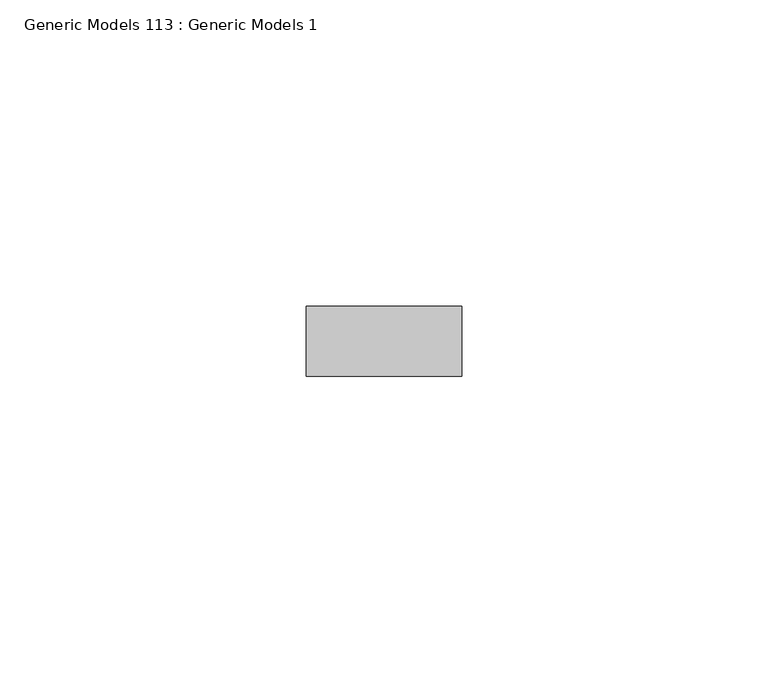
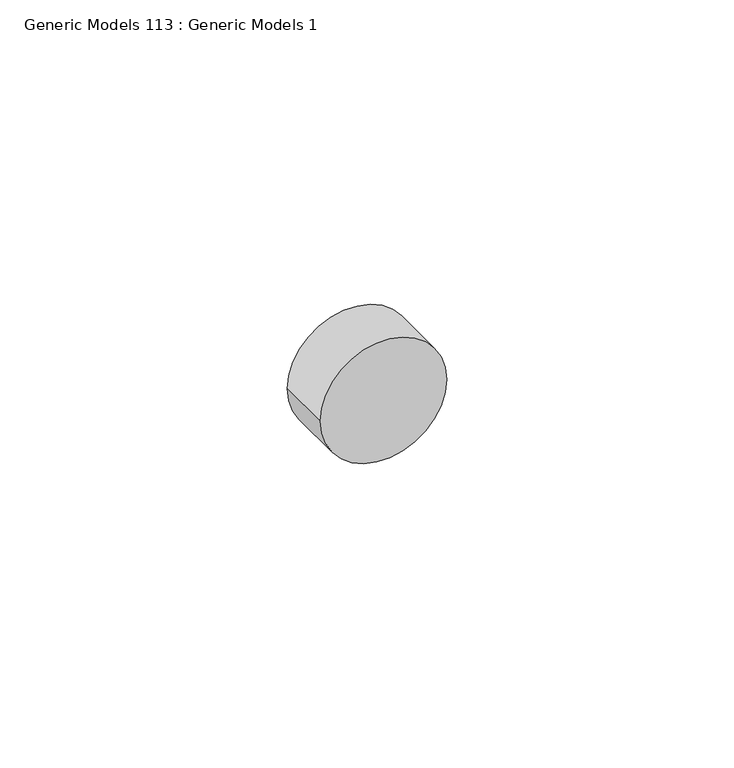
"""IFC4 building model written with IfcOpenShell, lengths in millimetres: proxy geometry, Generic Models 113 : Generic Models 1."""

from ifc_helpers import new_model, si_unit, point, frame, frame_2d, origin, place, context, project, spatial, circle_curve, trimmed, segment, composite_curve, outline, extrude, source, transform, mapped, element, save


def generic_models_113_generic_models_1_33cf204b(model_context):
    return source(origin(), model_context, "Body", "SweptSolid", [
        extrude(outline(composite_curve([segment(trimmed(circle_curve(frame_2d((37860.4162436, 6848.7828124)), 12.7), [point((37860.4162436, 6836.0828124))], [point((37860.4162436, 6861.4828124))], False, "CARTESIAN"), True, "CONTINUOUS"), segment(trimmed(circle_curve(frame_2d((37860.4162436, 6848.7828124)), 12.7), [point((37860.4162436, 6861.4828124))], [point((37860.4162436, 6836.0828124))], False, "CARTESIAN"), True, "CONTINUOUS")], self_intersect=False)), frame((0.0, 1836.9202358, 0.0), z_axis=(0.0, 1.0, 0.0), x_axis=(0.0, 0.0, 1.0)), (0.0, 0.0, 1.0), 11.4464372),
    ])


if __name__ == "__main__":
    model = new_model("IFC4")
    model_context = context("Model", 3, world=origin())
    ifc_project = project(units=[si_unit("LENGTHUNIT", "METRE", prefix="MILLI")], contexts=[model_context])
    site = spatial("IfcSite", under=ifc_project)
    building = spatial("IfcBuilding", under=site)
    placement = place(None, origin())
    generic_models_113_generic_models_1_shape = generic_models_113_generic_models_1_33cf204b(model_context)
    element("IfcBuildingElementProxy", 1, Name="Generic Models 113 : Generic Models 1", ObjectType="Generic Models 113 : Generic Models 1", at=placement, inside=building, context=model_context, shape_type="MappedRepresentation", body=[
        mapped(generic_models_113_generic_models_1_shape, transform((0.0, 0.0, 0.0), x_axis=(1.0, 0.0, 0.0), y_axis=(0.0, 1.0, 0.0), z_axis=(0.0, 0.0, 1.0))),
    ])
    save(model, "model.ifc")

# Revit data of these elements
# Element 1 (IfcBuildingElementProxy, "Generic Models 113 : Generic Models 1")
#   Materials on its faces: "S.S. LAG BOLT - SEE STRUCT. DWGS"
# Materials
#   "S.S. LAG BOLT - SEE STRUCT. DWGS": class "Generic", colour RGB 120 120 120, transparency 0, Cost = 0
